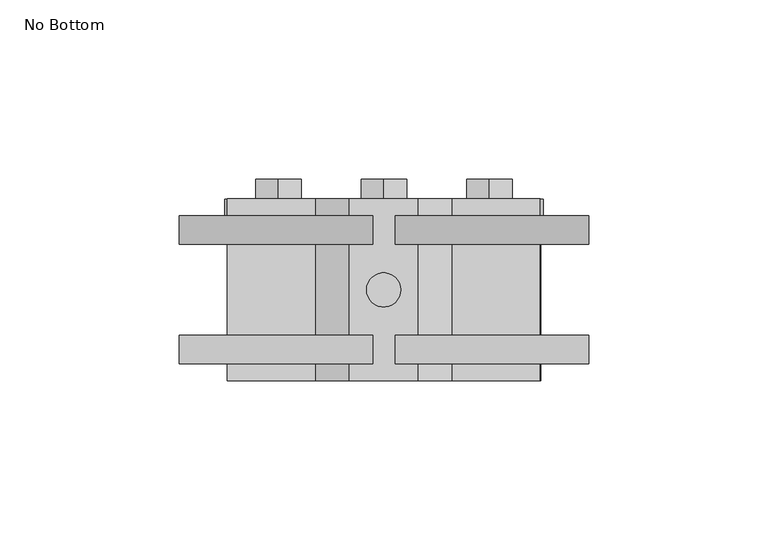
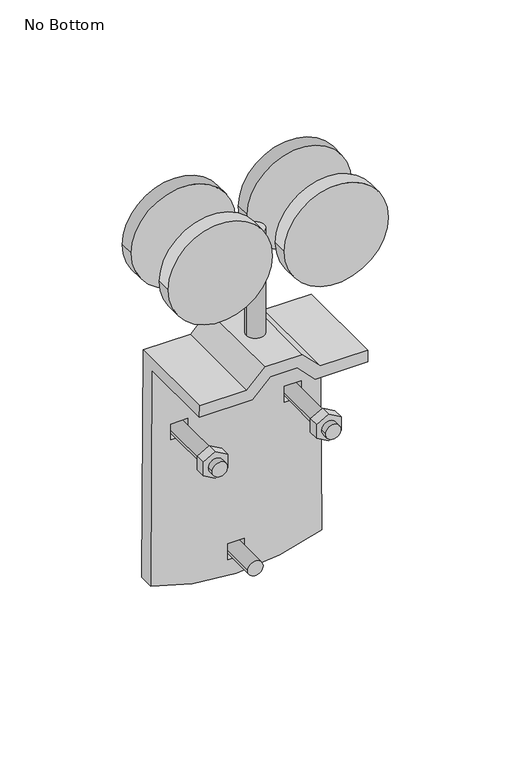
"""IFC4 building model written with IfcOpenShell, lengths in millimetres: proxy geometry, 087100_14 - Sliding and Folding Door Hardware - 5040 Box Rail Hangers : No Bottom."""

from ifc_helpers import new_model, si_unit, point, frame, frame_2d, origin, origin_with_axes, place, context, project, spatial, polyline, circle_curve, trimmed, segment, composite_curve, outline, extrude, source, transform, mapped, element, save
from ifc_brep_helpers import plane_surface, cylinder_surface, advanced_brep


def no_bottom_081a9404(model_context):
    return source(origin(), model_context, "Body", "SolidModel", [
        extrude(outline(polyline([(-110.0557037, -6.35), (-117.3880521, -6.35), (-121.0542263, 0.0), (-117.3880521, 6.35), (-110.0557037, 6.35), (-106.3895295, 0.0), (-110.0557037, -6.35)])), frame((0.0, 25.4, 0.0), z_axis=(0.0, 1.0, 0.0), x_axis=(0.0, 0.0, 1.0)), (0.0, 0.0, 1.0), 5.55625),
        extrude(outline(composite_curve([segment(trimmed(circle_curve(frame_2d((-113.7218779, 0.0)), 3.96875), [point((-113.7218779, -3.96875))], [point((-113.7218779, 3.96875))], False, "CARTESIAN"), True, "CONTINUOUS"), segment(trimmed(circle_curve(frame_2d((-113.7218779, 0.0)), 3.96875), [point((-113.7218779, 3.96875))], [point((-113.7218779, -3.96875))], False, "CARTESIAN"), True, "CONTINUOUS")], self_intersect=False)), frame((0.0, 0.0, 0.0), z_axis=(0.0, 1.0, 0.0), x_axis=(0.0, 0.0, 1.0)), (0.0, 0.0, 1.0), 25.4),
        extrude(outline(polyline([(-41.151956, -35.8279106), (-44.8181303, -29.4779106), (-41.151956, -23.1279106), (-33.8196076, -23.1279106), (-30.1534334, -29.4779106), (-33.8196076, -35.8279106), (-41.151956, -35.8279106)])), frame((0.0, -15.08125, 0.0), z_axis=(0.0, 1.0, 0.0), x_axis=(0.0, 0.0, 1.0)), (0.0, 0.0, 1.0), 5.55625),
        extrude(outline(polyline([(-33.8196076, -35.8279106), (-41.151956, -35.8279106), (-44.8181303, -29.4779106), (-41.151956, -23.1279106), (-33.8196076, -23.1279106), (-30.1534334, -29.4779106), (-33.8196076, -35.8279106)])), frame((0.0, 25.4, 0.0), z_axis=(0.0, 1.0, 0.0), x_axis=(0.0, 0.0, 1.0)), (0.0, 0.0, 1.0), 5.55625),
        extrude(outline(composite_curve([segment(trimmed(circle_curve(frame_2d((-37.4857818, -29.4779106)), 3.96875), [point((-37.4857818, -33.4466606))], [point((-37.4857818, -25.5091606))], False, "CARTESIAN"), True, "CONTINUOUS"), segment(trimmed(circle_curve(frame_2d((-37.4857818, -29.4779106)), 3.96875), [point((-37.4857818, -25.5091606))], [point((-37.4857818, -33.4466606))], False, "CARTESIAN"), True, "CONTINUOUS")], self_intersect=False)), frame((0.0, -19.05, 0.0), z_axis=(0.0, 1.0, 0.0), x_axis=(0.0, 0.0, 1.0)), (0.0, 0.0, 1.0), 44.45),
        extrude(outline(polyline([(-41.151956, 23.1279765), (-44.8181303, 29.4779765), (-41.151956, 35.8279765), (-33.8196076, 35.8279765), (-30.1534334, 29.4779765), (-33.8196076, 23.1279765), (-41.151956, 23.1279765)])), frame((0.0, -15.08125, 0.0), z_axis=(0.0, 1.0, 0.0), x_axis=(0.0, 0.0, 1.0)), (0.0, 0.0, 1.0), 5.55625),
        extrude(outline(polyline([(-33.8196076, 23.1279765), (-41.151956, 23.1279765), (-44.8181303, 29.4779765), (-41.151956, 35.8279765), (-33.8196076, 35.8279765), (-30.1534334, 29.4779765), (-33.8196076, 23.1279765)])), frame((0.0, 25.4, 0.0), z_axis=(0.0, 1.0, 0.0), x_axis=(0.0, 0.0, 1.0)), (0.0, 0.0, 1.0), 5.55625),
        extrude(outline(composite_curve([segment(trimmed(circle_curve(frame_2d((-37.4857818, 29.4779765)), 3.96875), [point((-37.4857818, 25.5092265))], [point((-37.4857818, 33.4467265))], False, "CARTESIAN"), True, "CONTINUOUS"), segment(trimmed(circle_curve(frame_2d((-37.4857818, 29.4779765)), 3.96875), [point((-37.4857818, 33.4467265))], [point((-37.4857818, 25.5092265))], False, "CARTESIAN"), True, "CONTINUOUS")], self_intersect=False)), frame((0.0, -19.05, 0.0), z_axis=(0.0, 1.0, 0.0), x_axis=(0.0, 0.0, 1.0)), (0.0, 0.0, 1.0), 44.45),
        advanced_brep(
        [(-44.4707374, 25.4, -118.5726247), (-43.7119983, 25.4, 6.35), (-19.059057, 25.4, 6.35), (-9.6566784, 25.4, 15.7523786), (9.6563712, 25.4, 15.7523786), (19.0589621, 25.4, 6.35), (43.7118564, 25.4, 6.35), (44.4707374, 25.4, -118.5726247), (-25.119743, 25.4, -33.1275483), (-33.8360782, 25.4, -33.1275483), (-33.8360782, 25.4, -41.8440154), (-25.119743, 25.4, -41.8440154), (33.8360782, 25.4, -33.1275483), (25.1198748, 25.4, -33.1275483), (25.1198748, 25.4, -41.8440154), (33.8360782, 25.4, -41.8440154), (4.3581017, 25.4, -109.3636444), (-4.3581017, 25.4, -109.3636444), (-4.3581017, 25.4, -118.0801114), (4.3581017, 25.4, -118.0801114), (-43.7119983, -25.4, 6.35), (-43.7505662, -25.4, 0.0), (-16.4288009, -25.4, 0.0), (-7.0264223, -25.4, 9.4023786), (7.0261571, -25.4, 9.4023786), (16.428748, -25.4, 0.0), (43.7504315, -25.4, 0.0), (43.7118564, -25.4, 6.35), (19.0589621, -25.4, 6.35), (9.6563712, -25.4, 15.7523786), (-9.6566784, -25.4, 15.7523786), (-19.059057, -25.4, 6.35), (-44.4707374, 17.4625, -118.5726247), (-43.7505662, 17.4625, 0.0), (-16.4288009, 17.4625, 0.0), (-7.0264223, 17.4625, 9.4023786), (7.0261571, 17.4625, 9.4023786), (16.428748, 17.4625, 0.0), (43.7504315, 17.4625, 0.0), (44.4707374, 17.4625, -118.5726247), (19.0589621, 17.4625, 6.35), (9.6563712, 17.4625, 15.7523786), (-9.6566784, 17.4625, 15.7523786), (-19.059057, 17.4625, 6.35), (-25.119743, 17.4625, -33.1275483), (-25.119743, 17.4625, -41.8440154), (-33.8360782, 17.4625, -41.8440154), (-33.8360782, 17.4625, -33.1275483), (33.8360782, 17.4625, -33.1275483), (33.8360782, 17.4625, -41.8440154), (25.1198748, 17.4625, -41.8440154), (25.1198748, 17.4625, -33.1275483), (4.3581017, 17.4625, -109.3636444), (4.3581017, 17.4625, -118.0801114), (-4.3581017, 17.4625, -118.0801114), (-4.3581017, 17.4625, -109.3636444)],
        [
            (0, 1),
            (1, 2),
            (2, 3),
            (3, 4),
            (4, 5),
            (5, 6),
            (6, 7),
            (7, 0, circle_curve(frame((0.0, 25.4, -6.3557626), z_axis=(0.0, 1.0, 0.0), x_axis=(1.0, 0.0, 0.0)), 120.7073761)),
            (8, 9),
            (9, 10),
            (10, 11),
            (11, 8),
            (12, 13),
            (13, 14),
            (14, 15),
            (15, 12),
            (16, 17),
            (17, 18),
            (18, 19),
            (19, 16),
            (20, 21),
            (21, 22),
            (22, 23),
            (23, 24),
            (24, 25),
            (25, 26),
            (26, 27),
            (27, 28),
            (28, 29),
            (29, 30),
            (30, 31),
            (31, 20),
            (0, 32),
            (32, 33),
            (33, 21),
            (20, 1),
            (33, 34),
            (34, 22),
            (34, 35),
            (35, 23),
            (35, 36),
            (36, 24),
            (36, 37),
            (37, 25),
            (37, 38),
            (38, 26),
            (6, 27),
            (38, 39),
            (39, 7),
            (5, 40),
            (40, 28),
            (4, 41),
            (41, 29),
            (3, 42),
            (42, 30),
            (2, 43),
            (43, 31),
            (32, 39, circle_curve(frame((0.0, 17.4625, -6.3557626), z_axis=(0.0, -1.0, 0.0), x_axis=(1.0, 0.0, 0.0)), 120.7073761)),
            (44, 45),
            (45, 46),
            (46, 47),
            (47, 44),
            (48, 49),
            (49, 50),
            (50, 51),
            (51, 48),
            (52, 53),
            (53, 54),
            (54, 55),
            (55, 52),
            (11, 45),
            (44, 8),
            (10, 46),
            (9, 47),
            (15, 49),
            (48, 12),
            (14, 50),
            (13, 51),
            (19, 53),
            (52, 16),
            (18, 54),
            (17, 55),
        ],
        [
            plane_surface(frame((-46.969086, 25.4, -529.9133004), z_axis=(0.0, 1.0, 0.0), x_axis=(-0.006073560512695754, 0.0, -0.9999815557612544))),
            plane_surface(frame((-46.969086, -25.4, -529.9133004), z_axis=(0.0, -1.0, 0.0), x_axis=(0.006073560512695754, 0.0, 0.9999815557612544))),
            plane_surface(frame((-43.7119983, 25.4, 6.35), z_axis=(-0.9999815557612544, 0.0, 0.006073560512695754), x_axis=(0.0, -1.0, 0.0))),
            plane_surface(frame((-43.7505662, 25.4, 0.0), z_axis=(0.0, 0.0, -1.0), x_axis=(0.0, -1.0, 0.0))),
            plane_surface(frame((-16.4288009, 25.4, 0.0), z_axis=(0.7071067811865476, 0.0, -0.7071067811865476), x_axis=(0.0, -1.0, 0.0))),
            plane_surface(frame((-7.0264223, 25.4, 9.4023786), z_axis=(0.0, 0.0, -1.0), x_axis=(0.0, -1.0, 0.0))),
            plane_surface(frame((7.0261571, 25.4, 9.4023786), z_axis=(-0.7070987963768838, 0.0, -0.7071147659060459), x_axis=(0.0, -1.0, 0.0))),
            plane_surface(frame((16.428748, 25.4, 0.0), z_axis=(0.0, 0.0, -1.0), x_axis=(0.0, -1.0, 0.0))),
            plane_surface(frame((43.7504315, 25.4, 0.0), z_axis=(0.9999815488618892, 0.0, 0.006074696352680505), x_axis=(0.0, -1.0, 0.0))),
            plane_surface(frame((43.7118564, 25.4, 6.35), z_axis=(0.0, 0.0, 1.0), x_axis=(0.0, -1.0, 0.0))),
            plane_surface(frame((19.0589621, 25.4, 6.35), z_axis=(0.7070987963768809, 0.0, 0.7071147659060488), x_axis=(0.0, -1.0, 0.0))),
            plane_surface(frame((9.6563712, 25.4, 15.7523786), z_axis=(0.0, 0.0, 1.0), x_axis=(0.0, -1.0, 0.0))),
            plane_surface(frame((-9.6566784, 25.4, 15.7523786), z_axis=(-0.7071067811865457, 0.0, 0.7071067811865495), x_axis=(0.0, -1.0, 0.0))),
            plane_surface(frame((-19.059057, 25.4, 6.35), z_axis=(0.0, 0.0, 1.0), x_axis=(0.0, -1.0, 0.0))),
            plane_surface(frame((-46.969086, 17.4625, -529.9133004), z_axis=(0.0, -1.0, 0.0), x_axis=(0.006073560512693812, 0.0, 0.9999815557612544))),
            cylinder_surface(frame((0.0, 17.4625, -6.3557626), z_axis=(0.0, 1.0, 0.0), x_axis=(1.0, 0.0, 0.0)), 120.7073761),
            plane_surface(frame((-25.119743, 25.4, -33.1275483), z_axis=(-1.0, 0.0, 0.0), x_axis=(0.0, -1.0, 0.0))),
            plane_surface(frame((-25.119743, 25.4, -41.8440154), z_axis=(0.0, 0.0, 1.0), x_axis=(0.0, -1.0, 0.0))),
            plane_surface(frame((-33.8360782, 25.4, -41.8440154), z_axis=(1.0, 0.0, 0.0), x_axis=(0.0, -1.0, 0.0))),
            plane_surface(frame((-33.8360782, 25.4, -33.1275483), z_axis=(0.0, 0.0, -1.0), x_axis=(0.0, -1.0, 0.0))),
            plane_surface(frame((33.8360782, 25.4, -33.1275483), z_axis=(-1.0, 0.0, 0.0), x_axis=(0.0, -1.0, 0.0))),
            plane_surface(frame((33.8360782, 25.4, -41.8440154), z_axis=(0.0, 0.0, 1.0), x_axis=(0.0, -1.0, 0.0))),
            plane_surface(frame((25.1198748, 25.4, -41.8440154), z_axis=(1.0, 0.0, 0.0), x_axis=(0.0, -1.0, 0.0))),
            plane_surface(frame((25.1198748, 25.4, -33.1275483), z_axis=(0.0, 0.0, -1.0), x_axis=(0.0, -1.0, 0.0))),
            plane_surface(frame((4.3581017, 25.4, -109.3636444), z_axis=(-1.0, 0.0, 0.0), x_axis=(0.0, -1.0, 0.0))),
            plane_surface(frame((4.3581017, 25.4, -118.0801114), z_axis=(0.0, 0.0, 1.0), x_axis=(0.0, -1.0, 0.0))),
            plane_surface(frame((-4.3581017, 25.4, -118.0801114), z_axis=(1.0, 0.0, 0.0), x_axis=(0.0, -1.0, 0.0))),
            plane_surface(frame((-4.3581017, 25.4, -109.3636444), z_axis=(0.0, 0.0, -1.0), x_axis=(0.0, -1.0, 0.0))),
        ],
        [
            (0, [[1, 2, 3, 4, 5, 6, 7, 8], [9, 10, 11, 12], [13, 14, 15, 16], [17, 18, 19, 20]]),
            (1, [[21, 22, 23, 24, 25, 26, 27, 28, 29, 30, 31, 32]]),
            (2, [[33, 34, 35, -21, 36, -1]]),
            (3, [[-35, 37, 38, -22]]),
            (4, [[-38, 39, 40, -23]]),
            (5, [[-40, 41, 42, -24]]),
            (6, [[-42, 43, 44, -25]]),
            (7, [[-44, 45, 46, -26]]),
            (8, [[47, -27, -46, 48, 49, -7]]),
            (9, [[50, 51, -28, -47, -6]]),
            (10, [[52, 53, -29, -51, -50, -5]]),
            (11, [[54, 55, -30, -53, -52, -4]]),
            (12, [[56, 57, -31, -55, -54, -3]]),
            (13, [[-32, -57, -56, -2, -36]]),
            (14, [[-48, -45, -43, -41, -39, -37, -34, 58], [59, 60, 61, 62], [63, 64, 65, 66], [67, 68, 69, 70]]),
            (15, [[-49, -58, -33, -8]]),
            (16, [[71, -59, 72, -12]]),
            (17, [[73, -60, -71, -11]]),
            (18, [[74, -61, -73, -10]]),
            (19, [[-72, -62, -74, -9]]),
            (20, [[75, -63, 76, -16]]),
            (21, [[77, -64, -75, -15]]),
            (22, [[78, -65, -77, -14]]),
            (23, [[-76, -66, -78, -13]]),
            (24, [[79, -67, 80, -20]]),
            (25, [[81, -68, -79, -19]]),
            (26, [[82, -69, -81, -18]]),
            (27, [[-80, -70, -82, -17]]),
        ],
    ),
        extrude(outline(composite_curve([segment(trimmed(circle_curve(frame_2d((71.8251107, -30.1481535)), 27.0838855), [point((71.8251107, -57.232039))], [point((71.8251107, -3.0642681))], False, "CARTESIAN"), True, "CONTINUOUS"), segment(trimmed(circle_curve(frame_2d((71.8251107, -30.1481535)), 27.0838855), [point((71.8251107, -3.0642681))], [point((71.8251107, -57.232039))], False, "CARTESIAN"), True, "CONTINUOUS")], self_intersect=False)), frame((0.0, -20.6375, 0.0), z_axis=(0.0, 1.0, 0.0), x_axis=(0.0, 0.0, 1.0)), (0.0, 0.0, 1.0), 7.9375),
        extrude(outline(composite_curve([segment(trimmed(circle_curve(frame_2d((71.8251107, 30.2054611)), 27.0838855), [point((71.8251107, 3.1215756))], [point((71.8251107, 57.2893465))], False, "CARTESIAN"), True, "CONTINUOUS"), segment(trimmed(circle_curve(frame_2d((71.8251107, 30.2054611)), 27.0838855), [point((71.8251107, 57.2893465))], [point((71.8251107, 3.1215756))], False, "CARTESIAN"), True, "CONTINUOUS")], self_intersect=False)), frame((0.0, -20.6375, 0.0), z_axis=(0.0, 1.0, 0.0), x_axis=(0.0, 0.0, 1.0)), (0.0, 0.0, 1.0), 7.9375),
        extrude(outline(composite_curve([segment(trimmed(circle_curve(frame_2d((-0.0657734, 0.0)), 4.7625), [point((-4.8282734, 0.0))], [point((4.6967266, 0.0))], False, "CARTESIAN"), True, "CONTINUOUS"), segment(trimmed(circle_curve(frame_2d((-0.0657734, 0.0)), 4.7625), [point((4.6967266, 0.0))], [point((-4.8282734, 0.0))], False, "CARTESIAN"), True, "CONTINUOUS")], self_intersect=False)), origin_with_axes(), (0.0, 0.0, 1.0), 73.5534737),
        extrude(outline(composite_curve([segment(trimmed(circle_curve(frame_2d((71.8251107, -30.1481535)), 27.0838855), [point((71.8251107, -57.232039))], [point((71.8251107, -3.0642681))], False, "CARTESIAN"), True, "CONTINUOUS"), segment(trimmed(circle_curve(frame_2d((71.8251107, -30.1481535)), 27.0838855), [point((71.8251107, -3.0642681))], [point((71.8251107, -57.232039))], False, "CARTESIAN"), True, "CONTINUOUS")], self_intersect=False)), frame((0.0, 12.7, 0.0), z_axis=(0.0, 1.0, 0.0), x_axis=(0.0, 0.0, 1.0)), (0.0, 0.0, 1.0), 7.9375),
        extrude(outline(composite_curve([segment(trimmed(circle_curve(frame_2d((71.8251107, 30.2054611)), 27.0838855), [point((71.8251107, 3.1215756))], [point((71.8251107, 57.2893465))], False, "CARTESIAN"), True, "CONTINUOUS"), segment(trimmed(circle_curve(frame_2d((71.8251107, 30.2054611)), 27.0838855), [point((71.8251107, 57.2893465))], [point((71.8251107, 3.1215756))], False, "CARTESIAN"), True, "CONTINUOUS")], self_intersect=False)), frame((0.0, 12.7, 0.0), z_axis=(0.0, 1.0, 0.0), x_axis=(0.0, 0.0, 1.0)), (0.0, 0.0, 1.0), 7.9375),
    ])


if __name__ == "__main__":
    model = new_model("IFC4")
    model_context = context("Model", 3, world=origin())
    ifc_project = project(units=[si_unit("LENGTHUNIT", "METRE", prefix="MILLI")], contexts=[model_context])
    site = spatial("IfcSite", under=ifc_project)
    building = spatial("IfcBuilding", under=site)
    placement = place(None, origin())
    no_bottom_shape = no_bottom_081a9404(model_context)
    element("IfcBuildingElementProxy", 1, Name="087100_14 - Sliding and Folding Door Hardware - 5040 Box Rail Hangers : No Bottom", ObjectType="087100_14 - Sliding and Folding Door Hardware - 5040 Box Rail Hangers : No Bottom", at=placement, inside=building, context=model_context, shape_type="MappedRepresentation", body=[
        mapped(no_bottom_shape, transform((0.0, 0.0, 0.0), x_axis=(1.0, 0.0, 0.0), y_axis=(0.0, 1.0, 0.0), z_axis=(0.0, 0.0, 1.0))),
    ])
    save(model, "model.ifc")

# Revit data of these elements
# Type "087100_14 - Sliding and Folding Door Hardware - 5040 Box Rail Hangers : No Bottom"
#   Default Elevation = 4' - 0"
#   Left Bolt = element 2408420
#   Bracket Material = BOX RAIL HANGER W/ GALV. FASTNERS (NATIONAL 5040)
#   Bottom Bolt = element 2408421
# Element 1 (IfcBuildingElementProxy, "087100_14 - Sliding and Folding Door Hardware - 5040 Box Rail Hangers : No Bottom")
#   Materials on its faces: "STRUCTURAL BOLTS (PAINT TO MATCH STEEL FINISH)", "BOX RAIL HANGER W/ GALV. FASTNERS (NATIONAL 5040)"
# Materials
#   "BOX RAIL HANGER W/ GALV. FASTNERS (NATIONAL 5040)": class "Metal", colour RGB 199 199 199, transparency 0, Description = "Structural steel, ASTM A36 Grade B, mill finish", Cost = 0
#   "STRUCTURAL BOLTS (PAINT TO MATCH STEEL FINISH)": class "Generic", colour RGB 120 120 120, transparency 0, Cost = 0
